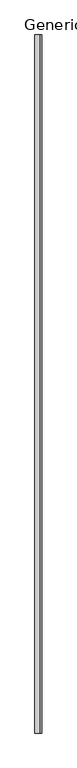
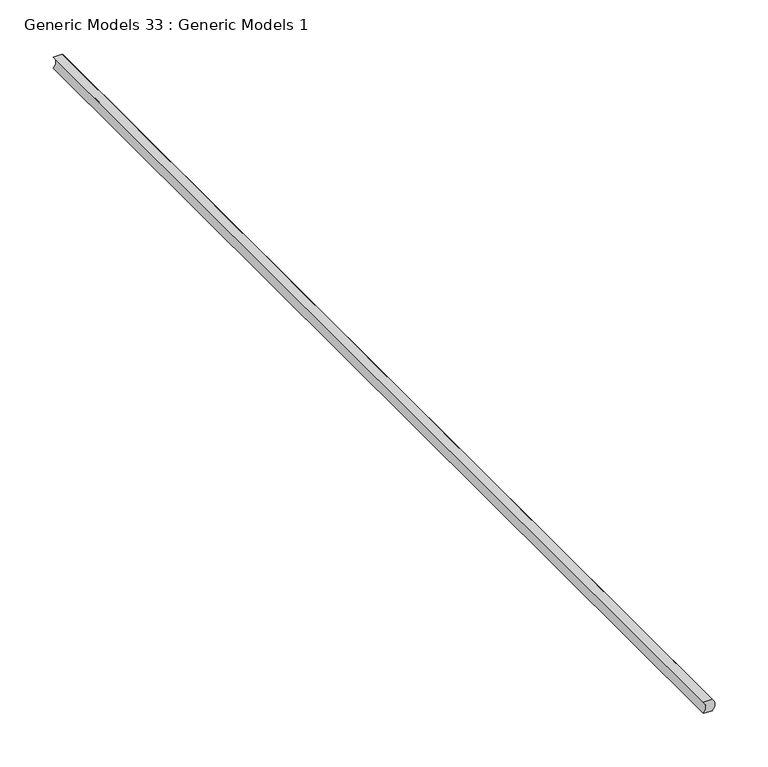
"""IFC4 building model written with IfcOpenShell, lengths in millimetres: proxy geometry, Generic Models 33 : Generic Models 1."""

from ifc_helpers import new_model, si_unit, point, frame, frame_2d, origin, place, context, project, spatial, polyline, circle_curve, trimmed, segment, composite_curve, outline, extrude, source, transform, mapped, element, save


def generic_models_33_generic_models_1_2dc3aaa3(model_context):
    return source(origin(), model_context, "Body", "SweptSolid", [
        extrude(outline(composite_curve([segment(polyline([(2444.75, 49676.05), (2444.75, 49685.575)]), True, "CONTINUOUS"), segment(trimmed(circle_curve(frame_2d((2451.1, 49679.745519)), 8.620055), [point((2444.75, 49685.575))], [point((2457.45, 49685.575))], False, "CARTESIAN"), True, "CONTINUOUS"), segment(polyline([(2457.45, 49685.575), (2457.45, 49676.05)]), True, "CONTINUOUS"), segment(trimmed(circle_curve(frame_2d((2451.1, 49670.220519)), 8.620055), [point((2457.45, 49676.05))], [point((2444.75, 49676.05))], True, "CARTESIAN"), True, "CONTINUOUS")], self_intersect=False)), frame((0.0, 0.0, 0.0), z_axis=(0.0, 1.0, 0.0), x_axis=(0.0, 0.0, 1.0)), (0.0, 0.0, 1.0), 1219.2),
    ])


if __name__ == "__main__":
    model = new_model("IFC4")
    model_context = context("Model", 3, world=origin())
    ifc_project = project(units=[si_unit("LENGTHUNIT", "METRE", prefix="MILLI")], contexts=[model_context])
    site = spatial("IfcSite", under=ifc_project)
    building = spatial("IfcBuilding", under=site)
    placement = place(None, origin())
    generic_models_33_generic_models_1_shape = generic_models_33_generic_models_1_2dc3aaa3(model_context)
    element("IfcBuildingElementProxy", 1, Name="Generic Models 33 : Generic Models 1", ObjectType="Generic Models 33 : Generic Models 1", at=placement, inside=building, context=model_context, shape_type="MappedRepresentation", body=[
        mapped(generic_models_33_generic_models_1_shape, transform((0.0, 0.0, 0.0), x_axis=(1.0, 0.0, 0.0), y_axis=(0.0, 1.0, 0.0), z_axis=(0.0, 0.0, 1.0))),
    ])
    save(model, "model.ifc")

# Revit data of these elements
# Element 1 (IfcBuildingElementProxy, "Generic Models 33 : Generic Models 1")
#   Materials on its faces: "ACOUSTICAL SEALANT"
# Materials
#   "ACOUSTICAL SEALANT": class "Unassigned", colour RGB 120 120 120, transparency 0, Cost = 0
